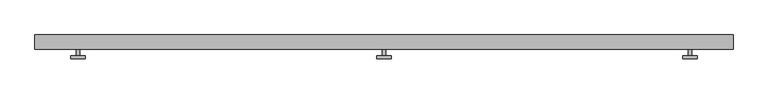
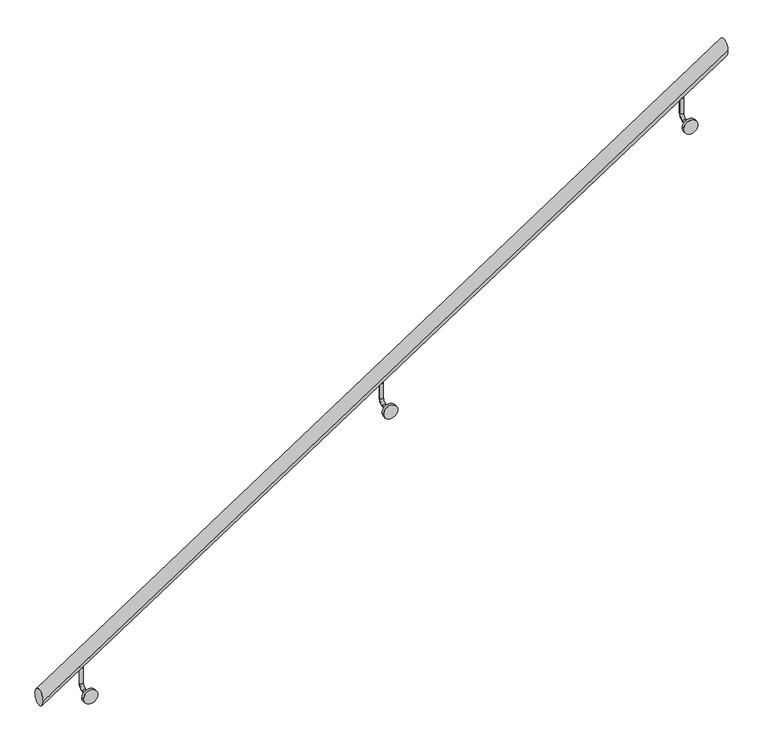
"""IFC4 building model written with IfcOpenShell, lengths in millimetres: railing geometry."""

import ifcopenshell
import ifcopenshell.guid

model = None  # the IFC model being written
_history = None  # IfcOwnerHistory: only IFC2X3 demands one
_inside = {}  # id of a spatial element -> (the spatial element, [elements in it])
_under = {}  # id of a project, library or spatial element -> (it, [spatial elements below it])
_declared = {}  # id of a project -> (the project, [libraries it declares])
_typed = {}  # id of a type object -> (the type object, [elements of that type])
_made_of = {}  # id of a material, layer set ... -> (it, [elements and type objects made of it])


def new_model(schema):
    """Start an empty IFC model of exactly this schema.

    Asked for "IFC4X3", IfcOpenShell would pick the latest addendum, in which some entities
    have other attributes; the version numbers below select the first issue.
    IFC2X3 requires an IfcOwnerHistory on every rooted entity: one is made here for all.
    """
    global model, _history
    if schema == "IFC4X3":
        model = ifcopenshell.file(schema_version=(4, 3, 0, 0))
    else:
        model = ifcopenshell.file(schema=schema)
    _inside.clear()
    _under.clear()
    _declared.clear()
    _typed.clear()
    _made_of.clear()
    _history = None
    if model.schema == "IFC2X3":
        org = make("IfcOrganization", Name="unknown")
        user = make(
            "IfcPersonAndOrganization",
            ThePerson=make("IfcPerson", FamilyName="unknown"),
            TheOrganization=org,
        )
        app = make(
            "IfcApplication",
            ApplicationDeveloper=org,
            Version="unknown",
            ApplicationFullName="unknown",
            ApplicationIdentifier="unknown",
        )
        _history = make(
            "IfcOwnerHistory",
            OwningUser=user,
            OwningApplication=app,
            ChangeAction="ADDED",
            CreationDate=0,
        )
    return model


def make(cls, **values):
    """One entity of the class cls with the attributes given. An attribute that is None is left unset."""
    return model.create_entity(
        cls, **{name: value for name, value in values.items() if value is not None}
    )


def rooted(cls, **values):
    """An entity with a GlobalId (a new one), such as an element, a storey or a relation."""
    return make(cls, GlobalId=ifcopenshell.guid.new(), OwnerHistory=_history, **values)


def si_unit(unit_type, name, prefix=None):
    """IfcSIUnit, for example si_unit("LENGTHUNIT", "METRE", prefix="MILLI")."""
    return make("IfcSIUnit", UnitType=unit_type, Prefix=prefix, Name=name)


def assignment(units):
    """IfcUnitAssignment: the units of a project."""
    return None if units is None else make("IfcUnitAssignment", Units=units)


def point(xyz):
    """IfcCartesianPoint."""
    return None if xyz is None else make("IfcCartesianPoint", Coordinates=xyz)


def direction(xyz):
    """IfcDirection."""
    return None if xyz is None else make("IfcDirection", DirectionRatios=xyz)


def frame(location, z_axis=None, x_axis=None):
    """IfcAxis2Placement3D, a coordinate frame: its origin and axes. An axis left out is left unset."""
    return make(
        "IfcAxis2Placement3D",
        Location=point(location),
        Axis=direction(z_axis),
        RefDirection=direction(x_axis),
    )


def frame_2d(location, x_axis=None):
    """IfcAxis2Placement2D, a coordinate frame in the plane: its origin and x axis."""
    return make(
        "IfcAxis2Placement2D", Location=point(location), RefDirection=direction(x_axis)
    )


def origin():
    """The frame at (0, 0, 0) with its axes left unset."""
    return frame((0.0, 0.0, 0.0))


def place(relative_to, where):
    """IfcLocalPlacement: puts the frame where relative to a parent placement (None: the world)."""
    return make(
        "IfcLocalPlacement", PlacementRelTo=relative_to, RelativePlacement=where
    )


def context(
    kind, dimensions, precision=None, world=None, true_north=None, identifier=None
):
    """IfcGeometricRepresentationContext, for example the 3D "Model" context."""
    return make(
        "IfcGeometricRepresentationContext",
        ContextIdentifier=identifier,
        ContextType=kind,
        CoordinateSpaceDimension=dimensions,
        Precision=precision,
        WorldCoordinateSystem=world,
        TrueNorth=true_north,
    )


def project(units=None, contexts=None):
    """IfcProject with its units and contexts."""
    return rooted(
        "IfcProject",
        Name="project",
        RepresentationContexts=contexts,
        UnitsInContext=assignment(units),
    )


def spatial(cls, under=None, at=None, **own):
    """A site, building, storey or space (cls), placed at a placement, below another one or the project."""
    s = rooted(cls, ObjectPlacement=at, **own)
    if under is not None:
        _under.setdefault(under.id(), (under, []))[1].append(s)
    return s


def circle_curve(where, radius):
    """IfcCircle in the frame where."""
    return make("IfcCircle", Position=where, Radius=radius)


def ellipse_curve(where, semi_axis1, semi_axis2):
    """IfcEllipse in the frame where."""
    return make(
        "IfcEllipse", Position=where, SemiAxis1=semi_axis1, SemiAxis2=semi_axis2
    )


def trimmed(basis, trim1, trim2, sense, master):
    """IfcTrimmedCurve: the piece of a basis curve between two trims."""
    return make(
        "IfcTrimmedCurve",
        BasisCurve=basis,
        Trim1=trim1,
        Trim2=trim2,
        SenseAgreement=sense,
        MasterRepresentation=master,
    )


def segment(curve, same_sense, transition):
    """IfcCompositeCurveSegment."""
    return make(
        "IfcCompositeCurveSegment",
        Transition=transition,
        SameSense=same_sense,
        ParentCurve=curve,
    )


def composite_curve(segments, self_intersect=None):
    """IfcCompositeCurve: segments joined end to end."""
    return make("IfcCompositeCurve", Segments=segments, SelfIntersect=self_intersect)


def outline(outer, holes=None, kind="AREA"):
    """IfcArbitraryClosedProfileDef: a profile drawn as a closed curve; with holes, ...WithVoids."""
    if holes is None:
        return make("IfcArbitraryClosedProfileDef", ProfileType=kind, OuterCurve=outer)
    return make(
        "IfcArbitraryProfileDefWithVoids",
        ProfileType=kind,
        OuterCurve=outer,
        InnerCurves=holes,
    )


def extrude(swept, where, along, depth):
    """IfcExtrudedAreaSolid: the profile swept, set in the frame where, extruded along a direction by depth."""
    return make(
        "IfcExtrudedAreaSolid",
        SweptArea=swept,
        Position=where,
        ExtrudedDirection=direction(along),
        Depth=depth,
    )


def shape(context_of_items, identifier, shape_type, items):
    """IfcShapeRepresentation: the items that make up one representation, for example the "Body"."""
    return make(
        "IfcShapeRepresentation",
        ContextOfItems=context_of_items,
        RepresentationIdentifier=identifier,
        RepresentationType=shape_type,
        Items=items,
    )


def source(mapping_origin, context_of_items, identifier, shape_type, items):
    """IfcRepresentationMap: a shape defined once, which mapped items show again and again."""
    return make(
        "IfcRepresentationMap",
        MappingOrigin=mapping_origin,
        MappedRepresentation=shape(context_of_items, identifier, shape_type, items),
    )


def transform(
    local_origin,
    x_axis=None,
    y_axis=None,
    z_axis=None,
    scale=None,
    scale2=None,
    scale3=None,
    uniform=True,
):
    """IfcCartesianTransformationOperator3D, or its non-uniform kind. x_axis, y_axis, z_axis: its Axis1, 2, 3."""
    if uniform:
        return make(
            "IfcCartesianTransformationOperator3D",
            Axis1=direction(x_axis),
            Axis2=direction(y_axis),
            LocalOrigin=point(local_origin),
            Scale=scale,
            Axis3=direction(z_axis),
        )
    return make(
        "IfcCartesianTransformationOperator3DnonUniform",
        Axis1=direction(x_axis),
        Axis2=direction(y_axis),
        LocalOrigin=point(local_origin),
        Scale=scale,
        Axis3=direction(z_axis),
        Scale2=scale2,
        Scale3=scale3,
    )


def mapped(mapping_source, mapping_target):
    """IfcMappedItem: shows the shape of a source again, moved by a transform."""
    return make(
        "IfcMappedItem", MappingSource=mapping_source, MappingTarget=mapping_target
    )


def made_of(thing, what):
    """Note that an element or type object is made of a material, layer set ...; save() writes the relation."""
    if what is not None:
        _made_of.setdefault(what.id(), (what, []))[1].append(thing)
    return thing


def element(
    cls,
    number,
    at=None,
    inside=None,
    cuts=None,
    type_object=None,
    material=None,
    context=None,
    identifier="Body",
    shape_type=None,
    held_by="IfcProductDefinitionShape",
    body=None,
    shapes=None,
    **own,
):
    """One element of the class cls, such as IfcWall. Its Tag is "e" and its number.

    at: its placement. inside: the storey or other place that contains it. cuts: it is an
    opening in that element (IfcRelVoidsElement). A single representation is given by context,
    identifier, shape_type and body (its items); several are given by shapes. held_by: the class
    of the entity that holds the representations. save() writes the other relations.
    """
    e = rooted(cls, Tag="e%d" % number, ObjectPlacement=at, **own)
    if body is not None:
        shapes = [shape(context, identifier, shape_type, body)]
    if shapes is not None:
        e.Representation = make(held_by, Representations=shapes)
    if inside is not None:
        _inside.setdefault(inside.id(), (inside, []))[1].append(e)
    if cuts is not None:
        rooted(
            "IfcRelVoidsElement", RelatingBuildingElement=cuts, RelatedOpeningElement=e
        )
    if type_object is not None:
        _typed.setdefault(type_object.id(), (type_object, []))[1].append(e)
    return made_of(e, material)


def aggregate(whole, parts):
    """IfcRelAggregates: a whole, such as a stair, and the parts it consists of."""
    return rooted("IfcRelAggregates", RelatingObject=whole, RelatedObjects=parts)


def save(model, path):
    """Write the relations noted so far, then the file.

    IfcRelAggregates (storeys below a building ...), IfcRelContainedInSpatialStructure (elements
    in a storey), IfcRelDefinesByType, IfcRelAssociatesMaterial and IfcRelDeclares: one each for
    every whole, place, type object, material and project.
    """
    for whole, parts in _under.values():
        aggregate(whole, parts)
    for where, things in _inside.values():
        rooted(
            "IfcRelContainedInSpatialStructure",
            RelatedElements=things,
            RelatingStructure=where,
        )
    for kind, things in _typed.values():
        rooted("IfcRelDefinesByType", RelatedObjects=things, RelatingType=kind)
    for what, things in _made_of.values():
        rooted("IfcRelAssociatesMaterial", RelatedObjects=things, RelatingMaterial=what)
    for by, libraries in _declared.values():
        rooted("IfcRelDeclares", RelatingContext=by, RelatedDefinitions=libraries)
    model.write(path)


def plane_surface(at):
    """IfcPlane: the flat surface through the origin of the frame at, square to its z axis."""
    return make("IfcPlane", Position=at)


def cylinder_surface(at, radius):
    """IfcCylindricalSurface: all points at the distance radius from the z axis of the frame at."""
    return make("IfcCylindricalSurface", Position=at, Radius=radius)


def revolved_surface(curve, axis_point, axis_direction):
    """IfcSurfaceOfRevolution: the curve turned about the line through axis_point along axis_direction."""
    return make(
        "IfcSurfaceOfRevolution",
        SweptCurve=make("IfcArbitraryOpenProfileDef", ProfileType="CURVE", Curve=curve),
        AxisPosition=make("IfcAxis1Placement", Location=point(axis_point), Axis=direction(axis_direction)),
    )


def advanced_brep(points, edges, surfaces, faces):
    """IfcAdvancedBrep: a solid bounded by faces that lie on surfaces and meet in shared edges.

    An edge is (start, end): straight between two places in points (the first is 0);
    or (start, end, curve); or (start, end, curve, False) where it runs against its curve.
    A face is (place in surfaces, loops), or (place, loops, False) where it looks against
    its surface's normal. A loop lists edges by number (the first is 1), with a minus sign
    where the edge is run from its end to its start. The first loop is the outer one.
    """
    corners = [point(p) for p in points]
    vertices = [make("IfcVertexPoint", VertexGeometry=c) for c in corners]
    made = []
    for start, end, *more in edges:
        made.append(
            make(
                "IfcEdgeCurve",
                EdgeStart=vertices[start],
                EdgeEnd=vertices[end],
                EdgeGeometry=more[0] if more else make("IfcPolyline", Points=[corners[start], corners[end]]),
                SameSense=more[1] if len(more) > 1 else True,
            )
        )
    hull = []
    for where, loops, *sense in faces:
        bounds = []
        for j, loop in enumerate(loops):
            ring = [make("IfcOrientedEdge", EdgeElement=made[abs(k) - 1], Orientation=k > 0) for k in loop]
            bounds.append(
                make(
                    "IfcFaceOuterBound" if j == 0 else "IfcFaceBound",
                    Bound=make("IfcEdgeLoop", EdgeList=ring),
                    Orientation=True,
                )
            )
        hull.append(make("IfcAdvancedFace", Bounds=bounds, FaceSurface=surfaces[where], SameSense=sense[0] if sense else True))
    return make("IfcAdvancedBrep", Outer=make("IfcClosedShell", CfsFaces=hull))


def railing_45cfc386(model_context):
    return source(origin(), model_context, "Body", "SolidModel", [
        advanced_brep(
        [(-50271.1127262, 15484.3574868, 2840.3133544), (-50271.1127262, 15434.3574868, 2840.3133544), (-47841.1127262, 15484.3574868, 4430.3133544), (-47841.1127262, 15434.3574868, 4430.3133544)],
        [
            (0, 1, ellipse_curve(frame((-50271.1127262, 15459.3574868, 2840.3133544), z_axis=(-1.0, 0.0, 0.0), x_axis=(0.0, 0.0, -1.0)), 29.8761606, 25.0)),
            (1, 0, ellipse_curve(frame((-50271.1127262, 15459.3574868, 2840.3133544), z_axis=(-1.0, 0.0, 0.0), x_axis=(0.0, 0.0, -1.0)), 29.8761606, 25.0)),
            (2, 3, ellipse_curve(frame((-47841.1127262, 15459.3574868, 4430.3133544), z_axis=(1.0, 0.0, 0.0), x_axis=(0.0, 0.0, -1.0)), 29.8761606, 25.0)),
            (3, 2, ellipse_curve(frame((-47841.1127262, 15459.3574868, 4430.3133544), z_axis=(1.0, 0.0, 0.0), x_axis=(0.0, 0.0, -1.0)), 29.8761606, 25.0)),
            (0, 2),
            (3, 1),
        ],
        [
            plane_surface(frame((-50271.1127262, 15459.3574868, 2870.189515), z_axis=(-1.0, 0.0, 0.0), x_axis=(0.0, 1.0, 0.0))),
            plane_surface(frame((-47841.1127262, 15459.3574868, 4460.189515), z_axis=(1.0, 0.0, 0.0), x_axis=(0.0, 1.0, 0.0))),
            cylinder_surface(frame((-50257.4245344, 15459.3574868, 2849.2698256), z_axis=(-0.8367875758947572, 0.0, -0.547527673116324), x_axis=(0.0, -1.0, 0.0)), 25.0),
        ],
        [
            (0, [[1, 2]]),
            (1, [[3, 4]]),
            (2, [[-1, 5, -4, 6]]),
            (2, [[-2, -6, -3, -5]]),
        ],
    ),
        advanced_brep(
        [(-49062.4627262, 15459.3574868, 3596.139515), (-49049.7627262, 15459.3574868, 3596.139515), (-49062.4627262, 15459.3574868, 3538.989515), (-49049.7627262, 15459.3574868, 3538.989515), (-49049.7627262, 15440.3074868, 3519.939515), (-49062.4627262, 15440.3074868, 3519.939515), (-49062.4627262, 15411.7324868, 3519.939515), (-49049.7627262, 15411.7324868, 3519.939515)],
        [
            (0, 1, circle_curve(frame((-49056.1127262, 15459.3574868, 3596.139515), z_axis=(0.0, 0.0, 1.0), x_axis=(1.0, 0.0, 0.0)), 6.35)),
            (1, 0, circle_curve(frame((-49056.1127262, 15459.3574868, 3596.139515), z_axis=(0.0, 0.0, 1.0), x_axis=(1.0, 0.0, 0.0)), 6.35)),
            (0, 2),
            (2, 3, circle_curve(frame((-49056.1127262, 15459.3574868, 3538.989515), z_axis=(0.0, 0.0, 1.0), x_axis=(1.0, 0.0, 0.0)), 6.35)),
            (3, 1),
            (3, 2, circle_curve(frame((-49056.1127262, 15459.3574868, 3538.989515), z_axis=(0.0, 0.0, 1.0), x_axis=(1.0, 0.0, 0.0)), 6.35)),
            (4, 3, circle_curve(frame((-49049.7627262, 15440.3074868, 3538.989515), z_axis=(1.0, 0.0, 0.0), x_axis=(0.0, 1.0, 0.0)), 19.05)),
            (2, 5, circle_curve(frame((-49062.4627262, 15440.3074868, 3538.989515), z_axis=(-1.0, 0.0, 0.0), x_axis=(0.0, 1.0, 0.0)), 19.05)),
            (5, 4, circle_curve(frame((-49056.1127262, 15440.3074868, 3519.939515), z_axis=(0.0, 1.0, 0.0), x_axis=(1.0, 0.0, 0.0)), 6.35)),
            (4, 5, circle_curve(frame((-49056.1127262, 15440.3074868, 3519.939515), z_axis=(0.0, 1.0, 0.0), x_axis=(1.0, 0.0, 0.0)), 6.35)),
            (6, 7, circle_curve(frame((-49056.1127262, 15411.7324868, 3519.939515), z_axis=(0.0, -1.0, 0.0), x_axis=(1.0, 0.0, 0.0)), 6.35)),
            (7, 6, circle_curve(frame((-49056.1127262, 15411.7324868, 3519.939515), z_axis=(0.0, -1.0, 0.0), x_axis=(1.0, 0.0, 0.0)), 6.35)),
            (5, 6),
            (7, 4),
        ],
        [
            plane_surface(frame((-49049.7627262, 15459.3574868, 3596.139515), z_axis=(0.0, 0.0, 1.0), x_axis=(0.0, -1.0, 0.0))),
            cylinder_surface(frame((-49056.1127262, 15459.3574868, 3596.139515), z_axis=(0.0, 0.0, 1.0), x_axis=(1.0, 0.0, 0.0)), 6.35),
            revolved_surface(trimmed(ellipse_curve(frame((-49056.1127262, 15459.3574868, 3538.989515), z_axis=(0.0, 0.0, 1.0), x_axis=(1.0, 0.0, 0.0)), 6.35, 6.35), [point((-49062.4627262, 15459.3574868, 3538.989515))], [point((-49049.7627262, 15459.3574868, 3538.989515))], True, "CARTESIAN"), (-49056.1127262, 15440.3074868, 3538.989515), (-1.0, 0.0, 0.0)),
            revolved_surface(trimmed(ellipse_curve(frame((-49056.1127262, 15459.3574868, 3538.989515), z_axis=(0.0, 0.0, 1.0), x_axis=(1.0, 0.0, 0.0)), 6.35, 6.35), [point((-49049.7627262, 15459.3574868, 3538.989515))], [point((-49062.4627262, 15459.3574868, 3538.989515))], True, "CARTESIAN"), (-49056.1127262, 15440.3074868, 3538.989515), (-1.0, 0.0, 0.0)),
            plane_surface(frame((-49056.1127262, 15411.7324868, 3513.589515), z_axis=(0.0, -1.0, 0.0), x_axis=(1.0, 0.0, 0.0))),
            cylinder_surface(frame((-49056.1127262, 15440.3074868, 3519.939515), z_axis=(0.0, 1.0, 0.0), x_axis=(1.0, 0.0, 0.0)), 6.35),
        ],
        [
            (0, [[1, 2]]),
            (1, [[-1, 3, 4, 5]]),
            (1, [[-2, -5, 6, -3]]),
            (2, [[7, -4, 8, 9]]),
            (3, [[-8, -6, -7, 10]]),
            (4, [[11, 12]]),
            (5, [[-9, 13, -12, 14]]),
            (5, [[-10, -14, -11, -13]]),
        ],
    ),
        extrude(outline(composite_curve([segment(trimmed(circle_curve(frame_2d((3519.939515, -49056.1127262)), 25.4), [point((3519.939515, -49030.7127262))], [point((3519.939515, -49081.5127262))], False, "CARTESIAN"), True, "CONTINUOUS"), segment(trimmed(circle_curve(frame_2d((3519.939515, -49056.1127262)), 25.4), [point((3519.939515, -49081.5127262))], [point((3519.939515, -49030.7127262))], False, "CARTESIAN"), True, "CONTINUOUS")], self_intersect=False)), frame((0.0, 15402.2074868, 0.0), z_axis=(0.0, 1.0, 0.0), x_axis=(0.0, 0.0, 1.0)), (0.0, 0.0, 1.0), 9.525),
        advanced_brep(
        [(-47997.4627262, 15459.3574868, 4292.9913669), (-47984.7627262, 15459.3574868, 4292.9913669), (-47997.4627262, 15459.3574868, 4235.8413669), (-47984.7627262, 15459.3574868, 4235.8413669), (-47984.7627262, 15440.3074868, 4216.7913669), (-47997.4627262, 15440.3074868, 4216.7913669), (-47997.4627262, 15411.7324868, 4216.7913669), (-47984.7627262, 15411.7324868, 4216.7913669)],
        [
            (0, 1, circle_curve(frame((-47991.1127262, 15459.3574868, 4292.9913669), z_axis=(0.0, 0.0, 1.0), x_axis=(1.0, 0.0, 0.0)), 6.35)),
            (1, 0, circle_curve(frame((-47991.1127262, 15459.3574868, 4292.9913669), z_axis=(0.0, 0.0, 1.0), x_axis=(1.0, 0.0, 0.0)), 6.35)),
            (0, 2),
            (2, 3, circle_curve(frame((-47991.1127262, 15459.3574868, 4235.8413669), z_axis=(0.0, 0.0, 1.0), x_axis=(1.0, 0.0, 0.0)), 6.35)),
            (3, 1),
            (3, 2, circle_curve(frame((-47991.1127262, 15459.3574868, 4235.8413669), z_axis=(0.0, 0.0, 1.0), x_axis=(1.0, 0.0, 0.0)), 6.35)),
            (4, 3, circle_curve(frame((-47984.7627262, 15440.3074868, 4235.8413669), z_axis=(1.0, 0.0, 0.0), x_axis=(0.0, 1.0, 0.0)), 19.05)),
            (2, 5, circle_curve(frame((-47997.4627262, 15440.3074868, 4235.8413669), z_axis=(-1.0, 0.0, 0.0), x_axis=(0.0, 1.0, 0.0)), 19.05)),
            (5, 4, circle_curve(frame((-47991.1127262, 15440.3074868, 4216.7913669), z_axis=(0.0, 1.0, 0.0), x_axis=(1.0, 0.0, 0.0)), 6.35)),
            (4, 5, circle_curve(frame((-47991.1127262, 15440.3074868, 4216.7913669), z_axis=(0.0, 1.0, 0.0), x_axis=(1.0, 0.0, 0.0)), 6.35)),
            (6, 7, circle_curve(frame((-47991.1127262, 15411.7324868, 4216.7913669), z_axis=(0.0, -1.0, 0.0), x_axis=(1.0, 0.0, 0.0)), 6.35)),
            (7, 6, circle_curve(frame((-47991.1127262, 15411.7324868, 4216.7913669), z_axis=(0.0, -1.0, 0.0), x_axis=(1.0, 0.0, 0.0)), 6.35)),
            (5, 6),
            (7, 4),
        ],
        [
            plane_surface(frame((-47984.7627262, 15459.3574868, 4292.9913669), z_axis=(0.0, 0.0, 1.0), x_axis=(0.0, -1.0, 0.0))),
            cylinder_surface(frame((-47991.1127262, 15459.3574868, 4292.9913669), z_axis=(0.0, 0.0, 1.0), x_axis=(1.0, 0.0, 0.0)), 6.35),
            revolved_surface(trimmed(ellipse_curve(frame((-47991.1127262, 15459.3574868, 4235.8413669), z_axis=(0.0, 0.0, 1.0), x_axis=(1.0, 0.0, 0.0)), 6.35, 6.35), [point((-47997.4627262, 15459.3574868, 4235.8413669))], [point((-47984.7627262, 15459.3574868, 4235.8413669))], True, "CARTESIAN"), (-47991.1127262, 15440.3074868, 4235.8413669), (-1.0, 0.0, 0.0)),
            revolved_surface(trimmed(ellipse_curve(frame((-47991.1127262, 15459.3574868, 4235.8413669), z_axis=(0.0, 0.0, 1.0), x_axis=(1.0, 0.0, 0.0)), 6.35, 6.35), [point((-47984.7627262, 15459.3574868, 4235.8413669))], [point((-47997.4627262, 15459.3574868, 4235.8413669))], True, "CARTESIAN"), (-47991.1127262, 15440.3074868, 4235.8413669), (-1.0, 0.0, 0.0)),
            plane_surface(frame((-47991.1127262, 15411.7324868, 4210.4413669), z_axis=(0.0, -1.0, 0.0), x_axis=(1.0, 0.0, 0.0))),
            cylinder_surface(frame((-47991.1127262, 15440.3074868, 4216.7913669), z_axis=(0.0, 1.0, 0.0), x_axis=(1.0, 0.0, 0.0)), 6.35),
        ],
        [
            (0, [[1, 2]]),
            (1, [[-1, 3, 4, 5]]),
            (1, [[-2, -5, 6, -3]]),
            (2, [[7, -4, 8, 9]]),
            (3, [[-8, -6, -7, 10]]),
            (4, [[11, 12]]),
            (5, [[-9, 13, -12, 14]]),
            (5, [[-10, -14, -11, -13]]),
        ],
    ),
        extrude(outline(composite_curve([segment(trimmed(circle_curve(frame_2d((4216.7913669, -47991.1127262)), 25.4), [point((4216.7913669, -47965.7127262))], [point((4216.7913669, -48016.5127262))], False, "CARTESIAN"), True, "CONTINUOUS"), segment(trimmed(circle_curve(frame_2d((4216.7913669, -47991.1127262)), 25.4), [point((4216.7913669, -48016.5127262))], [point((4216.7913669, -47965.7127262))], False, "CARTESIAN"), True, "CONTINUOUS")], self_intersect=False)), frame((0.0, 15402.2074868, 0.0), z_axis=(0.0, 1.0, 0.0), x_axis=(0.0, 0.0, 1.0)), (0.0, 0.0, 1.0), 9.525),
        advanced_brep(
        [(-50127.4627262, 15459.3574868, 2899.2876632), (-50114.7627262, 15459.3574868, 2899.2876632), (-50127.4627262, 15459.3574868, 2842.1376632), (-50114.7627262, 15459.3574868, 2842.1376632), (-50114.7627262, 15440.3074868, 2823.0876632), (-50127.4627262, 15440.3074868, 2823.0876632), (-50127.4627262, 15411.7324868, 2823.0876632), (-50114.7627262, 15411.7324868, 2823.0876632)],
        [
            (0, 1, circle_curve(frame((-50121.1127262, 15459.3574868, 2899.2876632), z_axis=(0.0, 0.0, 1.0), x_axis=(1.0, 0.0, 0.0)), 6.35)),
            (1, 0, circle_curve(frame((-50121.1127262, 15459.3574868, 2899.2876632), z_axis=(0.0, 0.0, 1.0), x_axis=(1.0, 0.0, 0.0)), 6.35)),
            (0, 2),
            (2, 3, circle_curve(frame((-50121.1127262, 15459.3574868, 2842.1376632), z_axis=(0.0, 0.0, 1.0), x_axis=(1.0, 0.0, 0.0)), 6.35)),
            (3, 1),
            (3, 2, circle_curve(frame((-50121.1127262, 15459.3574868, 2842.1376632), z_axis=(0.0, 0.0, 1.0), x_axis=(1.0, 0.0, 0.0)), 6.35)),
            (4, 3, circle_curve(frame((-50114.7627262, 15440.3074868, 2842.1376632), z_axis=(1.0, 0.0, 0.0), x_axis=(0.0, 1.0, 0.0)), 19.05)),
            (2, 5, circle_curve(frame((-50127.4627262, 15440.3074868, 2842.1376632), z_axis=(-1.0, 0.0, 0.0), x_axis=(0.0, 1.0, 0.0)), 19.05)),
            (5, 4, circle_curve(frame((-50121.1127262, 15440.3074868, 2823.0876632), z_axis=(0.0, 1.0, 0.0), x_axis=(1.0, 0.0, 0.0)), 6.35)),
            (4, 5, circle_curve(frame((-50121.1127262, 15440.3074868, 2823.0876632), z_axis=(0.0, 1.0, 0.0), x_axis=(1.0, 0.0, 0.0)), 6.35)),
            (6, 7, circle_curve(frame((-50121.1127262, 15411.7324868, 2823.0876632), z_axis=(0.0, -1.0, 0.0), x_axis=(1.0, 0.0, 0.0)), 6.35)),
            (7, 6, circle_curve(frame((-50121.1127262, 15411.7324868, 2823.0876632), z_axis=(0.0, -1.0, 0.0), x_axis=(1.0, 0.0, 0.0)), 6.35)),
            (5, 6),
            (7, 4),
        ],
        [
            plane_surface(frame((-50114.7627262, 15459.3574868, 2899.2876632), z_axis=(0.0, 0.0, 1.0), x_axis=(0.0, -1.0, 0.0))),
            cylinder_surface(frame((-50121.1127262, 15459.3574868, 2899.2876632), z_axis=(0.0, 0.0, 1.0), x_axis=(1.0, 0.0, 0.0)), 6.35),
            revolved_surface(trimmed(ellipse_curve(frame((-50121.1127262, 15459.3574868, 2842.1376632), z_axis=(0.0, 0.0, 1.0), x_axis=(1.0, 0.0, 0.0)), 6.35, 6.35), [point((-50127.4627262, 15459.3574868, 2842.1376632))], [point((-50114.7627262, 15459.3574868, 2842.1376632))], True, "CARTESIAN"), (-50121.1127262, 15440.3074868, 2842.1376632), (-1.0, 0.0, 0.0)),
            revolved_surface(trimmed(ellipse_curve(frame((-50121.1127262, 15459.3574868, 2842.1376632), z_axis=(0.0, 0.0, 1.0), x_axis=(1.0, 0.0, 0.0)), 6.35, 6.35), [point((-50114.7627262, 15459.3574868, 2842.1376632))], [point((-50127.4627262, 15459.3574868, 2842.1376632))], True, "CARTESIAN"), (-50121.1127262, 15440.3074868, 2842.1376632), (-1.0, 0.0, 0.0)),
            plane_surface(frame((-50121.1127262, 15411.7324868, 2816.7376632), z_axis=(0.0, -1.0, 0.0), x_axis=(1.0, 0.0, 0.0))),
            cylinder_surface(frame((-50121.1127262, 15440.3074868, 2823.0876632), z_axis=(0.0, 1.0, 0.0), x_axis=(1.0, 0.0, 0.0)), 6.35),
        ],
        [
            (0, [[1, 2]]),
            (1, [[-1, 3, 4, 5]]),
            (1, [[-2, -5, 6, -3]]),
            (2, [[7, -4, 8, 9]]),
            (3, [[-8, -6, -7, 10]]),
            (4, [[11, 12]]),
            (5, [[-9, 13, -12, 14]]),
            (5, [[-10, -14, -11, -13]]),
        ],
    ),
        extrude(outline(composite_curve([segment(trimmed(circle_curve(frame_2d((2823.0876632, -50121.1127262)), 25.4), [point((2823.0876632, -50095.7127262))], [point((2823.0876632, -50146.5127262))], False, "CARTESIAN"), True, "CONTINUOUS"), segment(trimmed(circle_curve(frame_2d((2823.0876632, -50121.1127262)), 25.4), [point((2823.0876632, -50146.5127262))], [point((2823.0876632, -50095.7127262))], False, "CARTESIAN"), True, "CONTINUOUS")], self_intersect=False)), frame((0.0, 15402.2074868, 0.0), z_axis=(0.0, 1.0, 0.0), x_axis=(0.0, 0.0, 1.0)), (0.0, 0.0, 1.0), 9.525),
    ])


if __name__ == "__main__":
    model = new_model("IFC4")
    model_context = context("Model", 3, world=origin())
    ifc_project = project(units=[si_unit("LENGTHUNIT", "METRE", prefix="MILLI")], contexts=[model_context])
    site = spatial("IfcSite", under=ifc_project)
    building = spatial("IfcBuilding", under=site)
    placement = place(None, origin())
    railing_shape = railing_45cfc386(model_context)
    element("IfcRailing", 1, at=placement, inside=building, context=model_context, shape_type="MappedRepresentation", body=[
        mapped(railing_shape, transform((0.0, 0.0, 0.0), x_axis=(1.0, 0.0, 0.0), y_axis=(0.0, 1.0, 0.0), z_axis=(0.0, 0.0, 1.0))),
    ])
    save(model, "model.ifc")
